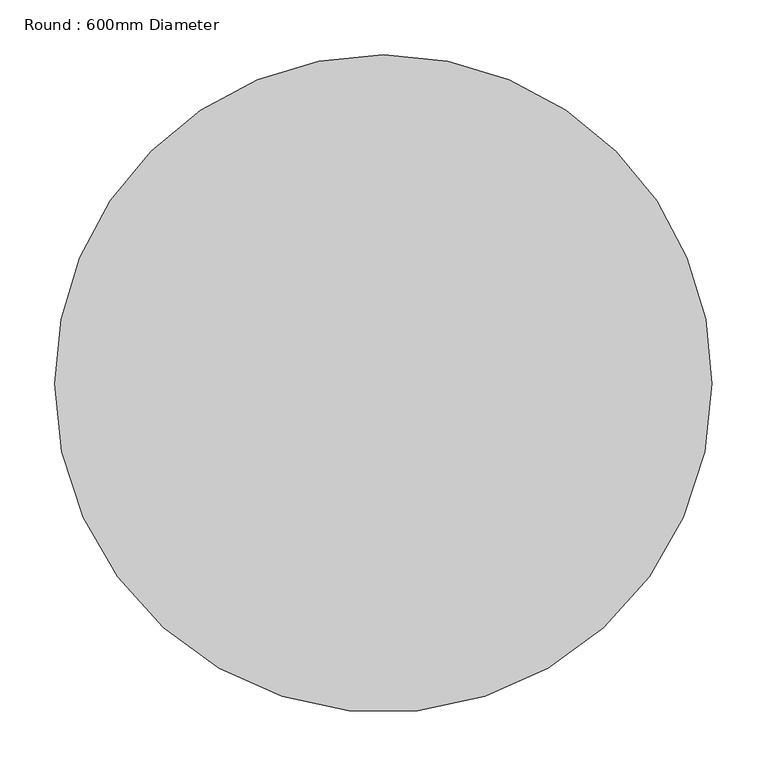
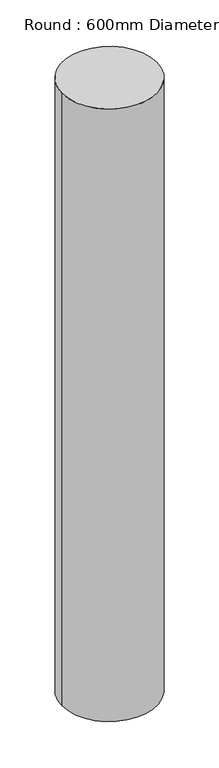
"""IFC4 building model written with IfcOpenShell, lengths in millimetres: column geometry, Round : 600mm Diameter."""

from ifc_helpers import new_model, si_unit, point, frame, origin, origin_2d, place, context, project, spatial, circle_curve, trimmed, segment, composite_curve, outline, extrude, source, transform, mapped, element, save


def round_600mm_diameter_eeded7df(model_context):
    return source(origin(), model_context, "Body", "SweptSolid", [
        extrude(outline(composite_curve([segment(trimmed(circle_curve(origin_2d(), 300.0), [point((300.0, 0.0))], [point((-300.0, 0.0))], False, "CARTESIAN"), True, "CONTINUOUS"), segment(trimmed(circle_curve(origin_2d(), 300.0), [point((-300.0, 0.0))], [point((0.0, 300.0))], False, "CARTESIAN"), True, "CONTINUOUS"), segment(trimmed(circle_curve(origin_2d(), 300.0), [point((0.0, 300.0))], [point((300.0, 0.0))], False, "CARTESIAN"), True, "CONTINUOUS")], self_intersect=False)), frame((0.0, 0.0, 138870.0), z_axis=(0.0, 0.0, 1.0), x_axis=(1.0, 0.0, 0.0)), (0.0, 0.0, 1.0), 4100.0),
    ])


if __name__ == "__main__":
    model = new_model("IFC4")
    model_context = context("Model", 3, world=origin())
    ifc_project = project(units=[si_unit("LENGTHUNIT", "METRE", prefix="MILLI")], contexts=[model_context])
    site = spatial("IfcSite", under=ifc_project)
    building = spatial("IfcBuilding", under=site)
    placement = place(None, origin())
    round_600mm_diameter_shape = round_600mm_diameter_eeded7df(model_context)
    element("IfcColumn", 1, ObjectType="Round : 600mm Diameter", at=placement, inside=building, context=model_context, shape_type="MappedRepresentation", body=[
        mapped(round_600mm_diameter_shape, transform((0.0, 0.0, 0.0), x_axis=(1.0, 0.0, 0.0), y_axis=(0.0, 1.0, 0.0), z_axis=(0.0, 0.0, 1.0))),
    ])
    save(model, "model.ifc")

# Revit data of these elements
# Type "Round : 600mm Diameter"
#   Keynote = "G"
#   Diameter = 600.00 mm
#   Offset Base = 0.00 mm
#   Offset Top = 0.00 mm
#   built-in parameter 1002110 = 8421504
#   built-in parameter 1002106 = element 3
#   Material = Concrete - Cast In Situ
# Element 1 (IfcColumn, "Round : 600mm Diameter")
#   Materials on its faces: "Concrete - Cast In Situ"
# Materials
#   "Concrete - Cast In Situ": class "Unassigned", colour RGB 255 255 255, transparency 0, Keynote = "E10/132", Cost = 0
